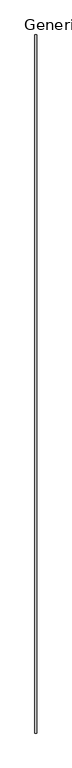
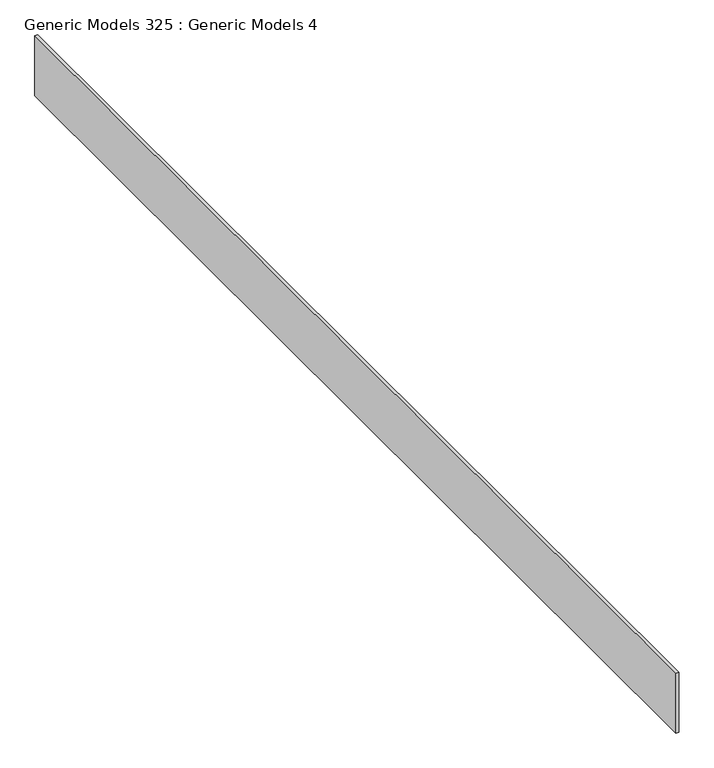
"""IFC4 building model written with IfcOpenShell, lengths in millimetres: proxy geometry, Generic Models 325 : Generic Models 4."""

from ifc_helpers import new_model, si_unit, frame, origin, place, context, project, spatial, polyline, outline, extrude, source, transform, mapped, element, save


def generic_models_325_generic_models_4_d98a1572(model_context):
    return source(origin(), model_context, "Body", "SweptSolid", [
        extrude(outline(polyline([(8331.3814682, -6864.9230338), (8315.5064682, -6864.9230338), (8315.5064682, -667.3230338), (8331.3814682, -667.3230338), (8331.3814682, -6864.9230338)])), frame((0.0, 0.0, 126361.8722633), z_axis=(0.0, 0.0, 1.0), x_axis=(1.0, 0.0, 0.0)), (0.0, 0.0, 1.0), 354.0125),
    ])


if __name__ == "__main__":
    model = new_model("IFC4")
    model_context = context("Model", 3, world=origin())
    ifc_project = project(units=[si_unit("LENGTHUNIT", "METRE", prefix="MILLI")], contexts=[model_context])
    site = spatial("IfcSite", under=ifc_project)
    building = spatial("IfcBuilding", under=site)
    placement = place(None, origin())
    generic_models_325_generic_models_4_shape = generic_models_325_generic_models_4_d98a1572(model_context)
    element("IfcBuildingElementProxy", 1, Name="Generic Models 325 : Generic Models 4", ObjectType="Generic Models 325 : Generic Models 4", at=placement, inside=building, context=model_context, shape_type="MappedRepresentation", body=[
        mapped(generic_models_325_generic_models_4_shape, transform((0.0, 0.0, 0.0), x_axis=(1.0, 0.0, 0.0), y_axis=(0.0, 1.0, 0.0), z_axis=(0.0, 0.0, 1.0))),
    ])
    save(model, "model.ifc")

# Revit data of these elements
# Element 1 (IfcBuildingElementProxy, "Generic Models 325 : Generic Models 4")
#   Materials on its faces: "_5/8\" DRYWALL"
# Materials
#   "_5/8\" DRYWALL": class "Generic", colour RGB 191 191 191, transparency 0, Cost = 0
